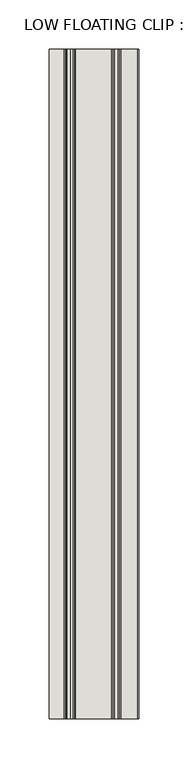
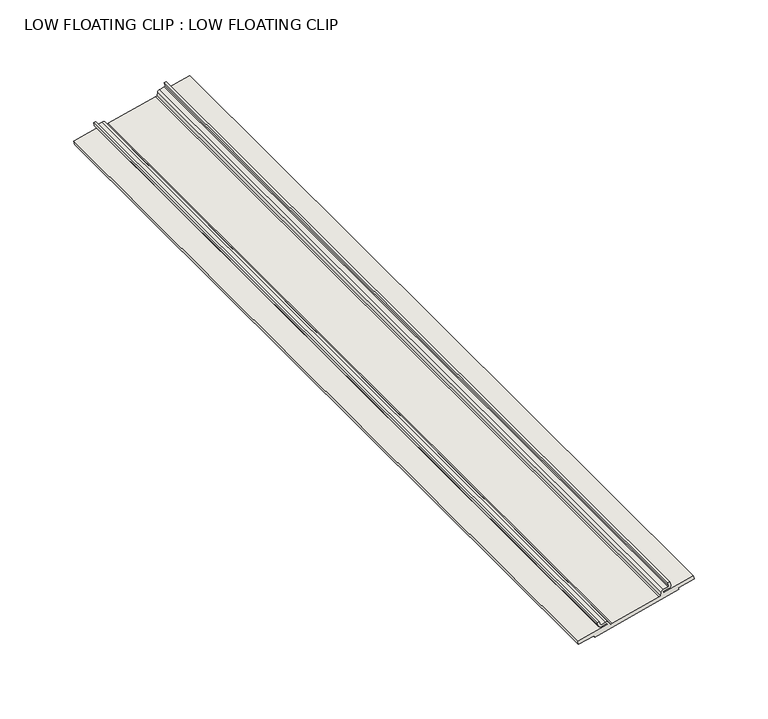
"""IFC4 building model written with IfcOpenShell, lengths in millimetres: wall geometry, LOW FLOATING CLIP : LOW FLOATING CLIP."""

import ifcopenshell
import ifcopenshell.guid

model = None  # the IFC model being written
_history = None  # IfcOwnerHistory: only IFC2X3 demands one
_inside = {}  # id of a spatial element -> (the spatial element, [elements in it])
_under = {}  # id of a project, library or spatial element -> (it, [spatial elements below it])
_declared = {}  # id of a project -> (the project, [libraries it declares])
_typed = {}  # id of a type object -> (the type object, [elements of that type])
_made_of = {}  # id of a material, layer set ... -> (it, [elements and type objects made of it])


def new_model(schema):
    """Start an empty IFC model of exactly this schema.

    Asked for "IFC4X3", IfcOpenShell would pick the latest addendum, in which some entities
    have other attributes; the version numbers below select the first issue.
    IFC2X3 requires an IfcOwnerHistory on every rooted entity: one is made here for all.
    """
    global model, _history
    if schema == "IFC4X3":
        model = ifcopenshell.file(schema_version=(4, 3, 0, 0))
    else:
        model = ifcopenshell.file(schema=schema)
    _inside.clear()
    _under.clear()
    _declared.clear()
    _typed.clear()
    _made_of.clear()
    _history = None
    if model.schema == "IFC2X3":
        org = make("IfcOrganization", Name="unknown")
        user = make(
            "IfcPersonAndOrganization",
            ThePerson=make("IfcPerson", FamilyName="unknown"),
            TheOrganization=org,
        )
        app = make(
            "IfcApplication",
            ApplicationDeveloper=org,
            Version="unknown",
            ApplicationFullName="unknown",
            ApplicationIdentifier="unknown",
        )
        _history = make(
            "IfcOwnerHistory",
            OwningUser=user,
            OwningApplication=app,
            ChangeAction="ADDED",
            CreationDate=0,
        )
    return model


def make(cls, **values):
    """One entity of the class cls with the attributes given. An attribute that is None is left unset."""
    return model.create_entity(
        cls, **{name: value for name, value in values.items() if value is not None}
    )


def rooted(cls, **values):
    """An entity with a GlobalId (a new one), such as an element, a storey or a relation."""
    return make(cls, GlobalId=ifcopenshell.guid.new(), OwnerHistory=_history, **values)


def si_unit(unit_type, name, prefix=None):
    """IfcSIUnit, for example si_unit("LENGTHUNIT", "METRE", prefix="MILLI")."""
    return make("IfcSIUnit", UnitType=unit_type, Prefix=prefix, Name=name)


def assignment(units):
    """IfcUnitAssignment: the units of a project."""
    return None if units is None else make("IfcUnitAssignment", Units=units)


def point(xyz):
    """IfcCartesianPoint."""
    return None if xyz is None else make("IfcCartesianPoint", Coordinates=xyz)


def direction(xyz):
    """IfcDirection."""
    return None if xyz is None else make("IfcDirection", DirectionRatios=xyz)


def frame(location, z_axis=None, x_axis=None):
    """IfcAxis2Placement3D, a coordinate frame: its origin and axes. An axis left out is left unset."""
    return make(
        "IfcAxis2Placement3D",
        Location=point(location),
        Axis=direction(z_axis),
        RefDirection=direction(x_axis),
    )


def origin():
    """The frame at (0, 0, 0) with its axes left unset."""
    return frame((0.0, 0.0, 0.0))


def place(relative_to, where):
    """IfcLocalPlacement: puts the frame where relative to a parent placement (None: the world)."""
    return make(
        "IfcLocalPlacement", PlacementRelTo=relative_to, RelativePlacement=where
    )


def context(
    kind, dimensions, precision=None, world=None, true_north=None, identifier=None
):
    """IfcGeometricRepresentationContext, for example the 3D "Model" context."""
    return make(
        "IfcGeometricRepresentationContext",
        ContextIdentifier=identifier,
        ContextType=kind,
        CoordinateSpaceDimension=dimensions,
        Precision=precision,
        WorldCoordinateSystem=world,
        TrueNorth=true_north,
    )


def project(units=None, contexts=None):
    """IfcProject with its units and contexts."""
    return rooted(
        "IfcProject",
        Name="project",
        RepresentationContexts=contexts,
        UnitsInContext=assignment(units),
    )


def spatial(cls, under=None, at=None, **own):
    """A site, building, storey or space (cls), placed at a placement, below another one or the project."""
    s = rooted(cls, ObjectPlacement=at, **own)
    if under is not None:
        _under.setdefault(under.id(), (under, []))[1].append(s)
    return s


def polyline(points):
    """IfcPolyline through the points."""
    return make("IfcPolyline", Points=[point(p) for p in points])


def circle_curve(where, radius):
    """IfcCircle in the frame where."""
    return make("IfcCircle", Position=where, Radius=radius)


def shape(context_of_items, identifier, shape_type, items):
    """IfcShapeRepresentation: the items that make up one representation, for example the "Body"."""
    return make(
        "IfcShapeRepresentation",
        ContextOfItems=context_of_items,
        RepresentationIdentifier=identifier,
        RepresentationType=shape_type,
        Items=items,
    )


def source(mapping_origin, context_of_items, identifier, shape_type, items):
    """IfcRepresentationMap: a shape defined once, which mapped items show again and again."""
    return make(
        "IfcRepresentationMap",
        MappingOrigin=mapping_origin,
        MappedRepresentation=shape(context_of_items, identifier, shape_type, items),
    )


def transform(
    local_origin,
    x_axis=None,
    y_axis=None,
    z_axis=None,
    scale=None,
    scale2=None,
    scale3=None,
    uniform=True,
):
    """IfcCartesianTransformationOperator3D, or its non-uniform kind. x_axis, y_axis, z_axis: its Axis1, 2, 3."""
    if uniform:
        return make(
            "IfcCartesianTransformationOperator3D",
            Axis1=direction(x_axis),
            Axis2=direction(y_axis),
            LocalOrigin=point(local_origin),
            Scale=scale,
            Axis3=direction(z_axis),
        )
    return make(
        "IfcCartesianTransformationOperator3DnonUniform",
        Axis1=direction(x_axis),
        Axis2=direction(y_axis),
        LocalOrigin=point(local_origin),
        Scale=scale,
        Axis3=direction(z_axis),
        Scale2=scale2,
        Scale3=scale3,
    )


def mapped(mapping_source, mapping_target):
    """IfcMappedItem: shows the shape of a source again, moved by a transform."""
    return make(
        "IfcMappedItem", MappingSource=mapping_source, MappingTarget=mapping_target
    )


def made_of(thing, what):
    """Note that an element or type object is made of a material, layer set ...; save() writes the relation."""
    if what is not None:
        _made_of.setdefault(what.id(), (what, []))[1].append(thing)
    return thing


def element(
    cls,
    number,
    at=None,
    inside=None,
    cuts=None,
    type_object=None,
    material=None,
    context=None,
    identifier="Body",
    shape_type=None,
    held_by="IfcProductDefinitionShape",
    body=None,
    shapes=None,
    **own,
):
    """One element of the class cls, such as IfcWall. Its Tag is "e" and its number.

    at: its placement. inside: the storey or other place that contains it. cuts: it is an
    opening in that element (IfcRelVoidsElement). A single representation is given by context,
    identifier, shape_type and body (its items); several are given by shapes. held_by: the class
    of the entity that holds the representations. save() writes the other relations.
    """
    e = rooted(cls, Tag="e%d" % number, ObjectPlacement=at, **own)
    if body is not None:
        shapes = [shape(context, identifier, shape_type, body)]
    if shapes is not None:
        e.Representation = make(held_by, Representations=shapes)
    if inside is not None:
        _inside.setdefault(inside.id(), (inside, []))[1].append(e)
    if cuts is not None:
        rooted(
            "IfcRelVoidsElement", RelatingBuildingElement=cuts, RelatedOpeningElement=e
        )
    if type_object is not None:
        _typed.setdefault(type_object.id(), (type_object, []))[1].append(e)
    return made_of(e, material)


def aggregate(whole, parts):
    """IfcRelAggregates: a whole, such as a stair, and the parts it consists of."""
    return rooted("IfcRelAggregates", RelatingObject=whole, RelatedObjects=parts)


def save(model, path):
    """Write the relations noted so far, then the file.

    IfcRelAggregates (storeys below a building ...), IfcRelContainedInSpatialStructure (elements
    in a storey), IfcRelDefinesByType, IfcRelAssociatesMaterial and IfcRelDeclares: one each for
    every whole, place, type object, material and project.
    """
    for whole, parts in _under.values():
        aggregate(whole, parts)
    for where, things in _inside.values():
        rooted(
            "IfcRelContainedInSpatialStructure",
            RelatedElements=things,
            RelatingStructure=where,
        )
    for kind, things in _typed.values():
        rooted("IfcRelDefinesByType", RelatedObjects=things, RelatingType=kind)
    for what, things in _made_of.values():
        rooted("IfcRelAssociatesMaterial", RelatedObjects=things, RelatingMaterial=what)
    for by, libraries in _declared.values():
        rooted("IfcRelDeclares", RelatingContext=by, RelatedDefinitions=libraries)
    model.write(path)


def plane_surface(at):
    """IfcPlane: the flat surface through the origin of the frame at, square to its z axis."""
    return make("IfcPlane", Position=at)


def cylinder_surface(at, radius):
    """IfcCylindricalSurface: all points at the distance radius from the z axis of the frame at."""
    return make("IfcCylindricalSurface", Position=at, Radius=radius)


def revolved_surface(curve, axis_point, axis_direction):
    """IfcSurfaceOfRevolution: the curve turned about the line through axis_point along axis_direction."""
    return make(
        "IfcSurfaceOfRevolution",
        SweptCurve=make("IfcArbitraryOpenProfileDef", ProfileType="CURVE", Curve=curve),
        AxisPosition=make("IfcAxis1Placement", Location=point(axis_point), Axis=direction(axis_direction)),
    )


def advanced_brep(points, edges, surfaces, faces):
    """IfcAdvancedBrep: a solid bounded by faces that lie on surfaces and meet in shared edges.

    An edge is (start, end): straight between two places in points (the first is 0);
    or (start, end, curve); or (start, end, curve, False) where it runs against its curve.
    A face is (place in surfaces, loops), or (place, loops, False) where it looks against
    its surface's normal. A loop lists edges by number (the first is 1), with a minus sign
    where the edge is run from its end to its start. The first loop is the outer one.
    """
    corners = [point(p) for p in points]
    vertices = [make("IfcVertexPoint", VertexGeometry=c) for c in corners]
    made = []
    for start, end, *more in edges:
        made.append(
            make(
                "IfcEdgeCurve",
                EdgeStart=vertices[start],
                EdgeEnd=vertices[end],
                EdgeGeometry=more[0] if more else make("IfcPolyline", Points=[corners[start], corners[end]]),
                SameSense=more[1] if len(more) > 1 else True,
            )
        )
    hull = []
    for where, loops, *sense in faces:
        bounds = []
        for j, loop in enumerate(loops):
            ring = [make("IfcOrientedEdge", EdgeElement=made[abs(k) - 1], Orientation=k > 0) for k in loop]
            bounds.append(
                make(
                    "IfcFaceOuterBound" if j == 0 else "IfcFaceBound",
                    Bound=make("IfcEdgeLoop", EdgeList=ring),
                    Orientation=True,
                )
            )
        hull.append(make("IfcAdvancedFace", Bounds=bounds, FaceSurface=surfaces[where], SameSense=sense[0] if sense else True))
    return make("IfcAdvancedBrep", Outer=make("IfcClosedShell", CfsFaces=hull))


def low_floating_clip_low_floating_clip_32a7baed(model_context):
    return source(origin(), model_context, "Body", "AdvancedBrep", [
        advanced_brep(
        [(19368.2427373, -2319.6634634, 2904.7050146), (19368.8587777, -2319.6634634, 2902.2408526), (19371.5072306, -2319.6634634, 2900.6517809), (19375.638583, -2319.6634634, 2901.684619), (19376.3038341, -2319.6634634, 2900.7867945), (19352.6994735, -2319.6634634, 2894.8857043), (19353.3982612, -2319.6634634, 2892.0905533), (19365.7199396, -2319.6634634, 2895.1709729), (19366.0898062, -2319.6634634, 2893.6915066), (19432.0053108, -2319.6634634, 2910.1703828), (19431.6354443, -2319.6634634, 2911.649849), (19443.9571227, -2319.6634634, 2914.7302686), (19443.2583349, -2319.6634634, 2917.5254197), (19419.6539743, -2319.6634634, 2911.6243295), (19419.8184549, -2319.6634634, 2912.729587), (19423.9498072, -2319.6634634, 2913.7624251), (19425.538879, -2319.6634634, 2916.410878), (19424.9228385, -2319.6634634, 2918.8750399), (19423.4448933, -2319.6634634, 2918.5055536), (19424.0609338, -2319.6634634, 2916.0413916), (19423.5794679, -2319.6634634, 2915.2397405), (19419.876029, -2319.6634634, 2914.3138808), (19418.244381, -2319.6634634, 2912.5153002), (19417.8358285, -2319.6634634, 2909.7698187), (19416.7891108, -2319.6634634, 2909.5081393), (19379.827509, -2319.6634634, 2900.2677388), (19378.7807913, -2319.6634634, 2900.0060594), (19377.1283125, -2319.6634634, 2902.236283), (19374.8422323, -2319.6634634, 2903.0554316), (19371.1387933, -2319.6634634, 2902.1295719), (19370.3372749, -2319.6634634, 2902.6104769), (19369.7206825, -2319.6634634, 2905.0745009), (19368.2427373, -1637.0384634, 2904.7050146), (19369.7206825, -1637.0384634, 2905.0745009), (19370.336723, -1637.0384634, 2902.610339), (19371.1387933, -1637.0384634, 2902.1295719), (19374.8422323, -1637.0384634, 2903.0554316), (19377.1283125, -1637.0384634, 2902.236283), (19378.7807913, -1637.0384634, 2900.0060594), (19379.827509, -1637.0384634, 2900.2677388), (19416.7891108, -1637.0384634, 2909.5081393), (19417.8358285, -1637.0384634, 2909.7698187), (19418.244381, -1637.0384634, 2912.5153002), (19419.876029, -1637.0384634, 2914.3138808), (19423.5794679, -1637.0384634, 2915.2397405), (19424.0603818, -1637.0384634, 2916.0412537), (19423.4448933, -1637.0384634, 2918.5055536), (19424.9228385, -1637.0384634, 2918.8750399), (19425.538879, -1637.0384634, 2916.410878), (19423.9498072, -1637.0384634, 2913.7624251), (19419.8184549, -1637.0384634, 2912.729587), (19419.6539743, -1637.0384634, 2911.6243295), (19443.2583349, -1637.0384634, 2917.5254197), (19443.9571227, -1637.0384634, 2914.7302686), (19431.6354443, -1637.0384634, 2911.649849), (19432.0053108, -1637.0384634, 2910.1703828), (19366.0898062, -1637.0384634, 2893.6915066), (19365.7199396, -1637.0384634, 2895.1709729), (19353.3982612, -1637.0384634, 2892.0905533), (19352.6994735, -1637.0384634, 2894.8857043), (19376.3038341, -1637.0384634, 2900.7867945), (19375.638583, -1637.0384634, 2901.684619), (19371.5072306, -1637.0384634, 2900.6517809), (19368.8587777, -1637.0384634, 2902.2408526)],
        [
            (0, 1),
            (1, 2, circle_curve(frame((19370.9775401, -2319.6634634, 2902.7705432), z_axis=(0.0, -1.0, 0.0), x_axis=(-0.9701425001453214, 0.0, -0.24253562503637516)), 2.1839702)),
            (2, 3),
            (3, 4),
            (4, 5),
            (5, 6),
            (6, 7),
            (7, 8),
            (8, 9),
            (9, 10),
            (10, 11),
            (11, 12),
            (12, 13),
            (13, 14),
            (14, 15),
            (15, 16, circle_curve(frame((19423.4201167, -2319.6634634, 2915.8811874), z_axis=(0.0, -1.0, 0.0), x_axis=(0.9701425001453399, 0.0, 0.2425356250363014)), 2.1839702)),
            (16, 17),
            (17, 18),
            (18, 19),
            (19, 20, circle_curve(frame((19423.4191639, -2319.6634634, 2915.8809567), z_axis=(0.0, 1.0, 0.0), x_axis=(0.2425356250361952, 0.0, -0.9701425001453665)), 0.6609505)),
            (20, 21),
            (21, 22, circle_curve(frame((19420.4060948, -2319.6634634, 2912.1936176), z_axis=(0.0, -1.0, 0.0), x_axis=(-0.9891084891577027, 0.0, 0.147188303462493)), 2.1855173)),
            (22, 23),
            (23, 24),
            (24, 25),
            (25, 26),
            (26, 27),
            (27, 28, circle_curve(frame((19375.3722981, -2319.6634634, 2900.9351684), z_axis=(0.0, -1.0, 0.0), x_axis=(0.8034777005685577, 0.0, 0.5953348508940689)), 2.1855173)),
            (28, 29),
            (29, 30, circle_curve(frame((19370.9784893, -2319.6634634, 2902.770788), z_axis=(0.0, 1.0, 0.0), x_axis=(0.2425356250364814, 0.0, -0.9701425001452949)), 0.6609505)),
            (30, 31),
            (31, 0),
            (32, 33),
            (33, 34),
            (34, 35, circle_curve(frame((19370.9784893, -1637.0384634, 2902.770788), z_axis=(0.0, -1.0, 0.0), x_axis=(0.2425356250364814, 0.0, -0.9701425001452949)), 0.6609505)),
            (35, 36),
            (36, 37, circle_curve(frame((19375.3722981, -1637.0384634, 2900.9351684), z_axis=(0.0, 1.0, 0.0), x_axis=(0.8034777005685577, 0.0, 0.5953348508940689)), 2.1855173)),
            (37, 38),
            (38, 39),
            (39, 40),
            (40, 41),
            (41, 42),
            (42, 43, circle_curve(frame((19420.4060948, -1637.0384634, 2912.1936176), z_axis=(0.0, 1.0, 0.0), x_axis=(-0.9891084891577027, 0.0, 0.147188303462493)), 2.1855173)),
            (43, 44),
            (44, 45, circle_curve(frame((19423.4191639, -1637.0384634, 2915.8809567), z_axis=(0.0, -1.0, 0.0), x_axis=(0.2425356250361952, 0.0, -0.9701425001453665)), 0.6609505)),
            (45, 46),
            (46, 47),
            (47, 48),
            (48, 49, circle_curve(frame((19423.4201167, -1637.0384634, 2915.8811874), z_axis=(0.0, 1.0, 0.0), x_axis=(0.9701425001453399, 0.0, 0.2425356250363014)), 2.1839702)),
            (49, 50),
            (50, 51),
            (51, 52),
            (52, 53),
            (53, 54),
            (54, 55),
            (55, 56),
            (56, 57),
            (57, 58),
            (58, 59),
            (59, 60),
            (60, 61),
            (61, 62),
            (62, 63, circle_curve(frame((19370.9775401, -1637.0384634, 2902.7705432), z_axis=(0.0, 1.0, 0.0), x_axis=(-0.9701425001453214, 0.0, -0.24253562503637516)), 2.1839702)),
            (63, 32),
            (0, 32),
            (63, 1),
            (62, 2),
            (61, 3),
            (60, 4),
            (59, 5),
            (58, 6),
            (57, 7),
            (56, 8),
            (55, 9),
            (54, 10),
            (53, 11),
            (52, 12),
            (51, 13),
            (50, 14),
            (49, 15),
            (48, 16),
            (47, 17),
            (46, 18),
            (45, 19),
            (44, 20),
            (43, 21),
            (42, 22),
            (41, 23),
            (40, 24),
            (39, 25),
            (38, 26),
            (37, 27),
            (36, 28),
            (35, 29),
            (34, 30),
            (33, 31),
        ],
        [
            plane_surface(frame((19368.2427373, -2319.6634634, 2904.7050146), z_axis=(0.0, -1.0, 0.0), x_axis=(0.24253562503683454, 0.0, -0.9701425001452065))),
            plane_surface(frame((19368.2427373, -1637.0384634, 2904.7050146), z_axis=(0.0, 1.0, 0.0), x_axis=(-0.24253562503683454, 0.0, 0.9701425001452065))),
            plane_surface(frame((19368.2427373, -2319.6634634, 2904.7050146), z_axis=(-0.9701425001452065, 0.0, -0.24253562503683454), x_axis=(0.0, 1.0, 0.0))),
            cylinder_surface(frame((19370.9775401, -1637.0384634, 2902.7705432), z_axis=(0.0, -1.0000000000000002, 0.0), x_axis=(-0.9701425001453214, 0.0, -0.24253562503637516)), 2.1839702),
            plane_surface(frame((19371.5072306, -2319.6634634, 2900.6517809), z_axis=(0.24253562520086946, 0.0, -0.9701425001041978), x_axis=(0.0, 1.0, 0.0))),
            plane_surface(frame((19375.638583, -2319.6634634, 2901.684619), z_axis=(-0.8034733269729771, 0.0, -0.5953407535546138), x_axis=(0.0, 1.0, 0.0))),
            plane_surface(frame((19376.3038341, -2319.6634634, 2900.7867945), z_axis=(-0.24253562503641676, 0.0, 0.970142500145311), x_axis=(0.0, 1.0, 0.0))),
            plane_surface(frame((19352.6994735, -2319.6634634, 2894.8857043), z_axis=(-0.9701425001452767, 0.0, -0.24253562503655407), x_axis=(0.0, 1.0, 0.0))),
            plane_surface(frame((19353.3982612, -2319.6634634, 2892.0905533), z_axis=(0.24253562503641324, 0.0, -0.9701425001453119), x_axis=(0.0, 1.0, 0.0))),
            plane_surface(frame((19365.7199396, -2319.6634634, 2895.1709729), z_axis=(-0.9701425001450604, 0.0, -0.242535625037419), x_axis=(0.0, 1.0, 0.0))),
            plane_surface(frame((19366.0898062, -2319.6634634, 2893.6915066), z_axis=(0.24253562503641551, 0.0, -0.9701425001453113), x_axis=(0.0, 1.0, 0.0))),
            plane_surface(frame((19432.0053108, -2319.6634634, 2910.1703828), z_axis=(0.9701425001452693, 0.0, 0.2425356250365836), x_axis=(0.0, 1.0, 0.0))),
            plane_surface(frame((19431.6354443, -2319.6634634, 2911.649849), z_axis=(0.24253562503625273, 0.0, -0.970142500145352), x_axis=(0.0, 1.0, 0.0))),
            plane_surface(frame((19443.9571227, -2319.6634634, 2914.7302686), z_axis=(0.9701425001452103, 0.0, 0.24253562503681939), x_axis=(0.0, 1.0, 0.0))),
            plane_surface(frame((19443.2583349, -2319.6634634, 2917.5254197), z_axis=(-0.24253562503627013, 0.0, 0.9701425001453476), x_axis=(0.0, 1.0, 0.0))),
            plane_surface(frame((19419.6539743, -2319.6634634, 2911.6243295), z_axis=(0.9891074078253219, 0.0, -0.14719556985545568), x_axis=(0.0, 1.0, 0.0))),
            plane_surface(frame((19419.8184549, -2319.6634634, 2912.729587), z_axis=(0.24253562503621331, 0.0, -0.9701425001453619), x_axis=(0.0, 1.0, 0.0))),
            cylinder_surface(frame((19423.4201167, -1637.0384634, 2915.8811874), z_axis=(0.0, -1.0000000000000002, 0.0), x_axis=(0.9701425001453399, 0.0, 0.2425356250363014)), 2.1839702),
            plane_surface(frame((19425.538879, -2319.6634634, 2916.410878), z_axis=(0.97014250014631, 0.0, 0.24253562503242082), x_axis=(0.0, 1.0, 0.0))),
            plane_surface(frame((19424.9228385, -2319.6634634, 2918.8750399), z_axis=(-0.24253562503633297, 0.0, 0.9701425001453319), x_axis=(0.0, 1.0, 0.0))),
            plane_surface(frame((19423.4448933, -2319.6634634, 2918.5055536), z_axis=(-0.9701425001454071, 0.0, -0.24253562503603204), x_axis=(0.0, 1.0, 0.0))),
            revolved_surface(polyline([(19423.579467942633, -1637.0384634, 2915.2397405294573), (19423.579467942633, -2319.6634634, 2915.2397405294573)]), (19423.4191639, -1637.0384634, 2915.8809567), (0.0, 1.0000000000000002, 0.0)),
            plane_surface(frame((19423.5794679, -2319.6634634, 2915.2397405), z_axis=(-0.242535625035799, 0.0, 0.9701425001454654), x_axis=(0.0, 1.0, 0.0))),
            cylinder_surface(frame((19420.4060948, -1637.0384634, 2912.1936176), z_axis=(0.0, -1.0, 0.0), x_axis=(-0.9891084891577027, 0.0, 0.147188303462493)), 2.1855173),
            plane_surface(frame((19418.244381, -2319.6634634, 2912.5153002), z_axis=(-0.9891084891587392, 0.0, 0.1471883034555279), x_axis=(0.0, 1.0, 0.0))),
            plane_surface(frame((19417.8358285, -2319.6634634, 2909.7698187), z_axis=(-0.24253562503586068, 0.0, 0.97014250014545), x_axis=(0.0, 1.0, 0.0))),
            plane_surface(frame((19416.7891108, -2319.6634634, 2909.5081393), z_axis=(-0.24253562503634635, 0.0, 0.9701425001453285), x_axis=(0.0, 1.0, 0.0))),
            plane_surface(frame((19379.827509, -2319.6634634, 2900.2677388), z_axis=(-0.24253562503633297, 0.0, 0.9701425001453319), x_axis=(0.0, 1.0, 0.0))),
            plane_surface(frame((19378.7807913, -2319.6634634, 2900.0060594), z_axis=(0.8034777005687778, 0.0, 0.5953348508937718), x_axis=(0.0, 1.0, 0.0))),
            cylinder_surface(frame((19375.3722981, -1637.0384634, 2900.9351684), z_axis=(0.0, -1.0000000000000002, 0.0), x_axis=(0.8034777005685577, 0.0, 0.5953348508940689)), 2.1855173),
            plane_surface(frame((19374.8422323, -2319.6634634, 2903.0554316), z_axis=(-0.24253562742045254, 0.0, 0.9701424995493021), x_axis=(0.0, 1.0, 0.0))),
            revolved_surface(polyline([(19371.138793342634, -1637.0384634, 2902.1295718294577), (19371.138793342634, -2319.6634634, 2902.1295718294577)]), (19370.9784893, -1637.0384634, 2902.770788), (0.0, 1.0000000000000002, 0.0)),
            plane_surface(frame((19370.336723, -2319.6634634, 2902.610339), z_axis=(0.9701425001453114, 0.0, 0.2425356250364152), x_axis=(0.0, 1.0, 0.0))),
            plane_surface(frame((19369.7206825, -2319.6634634, 2905.0745009), z_axis=(-0.24253562503633297, 0.0, 0.9701425001453319), x_axis=(0.0, 1.0, 0.0))),
        ],
        [
            (0, [[1, 2, 3, 4, 5, 6, 7, 8, 9, 10, 11, 12, 13, 14, 15, 16, 17, 18, 19, 20, 21, 22, 23, 24, 25, 26, 27, 28, 29, 30, 31, 32]]),
            (1, [[33, 34, 35, 36, 37, 38, 39, 40, 41, 42, 43, 44, 45, 46, 47, 48, 49, 50, 51, 52, 53, 54, 55, 56, 57, 58, 59, 60, 61, 62, 63, 64]]),
            (2, [[-1, 65, -64, 66]]),
            (3, [[-2, -66, -63, 67]]),
            (4, [[-3, -67, -62, 68]]),
            (5, [[-4, -68, -61, 69]]),
            (6, [[-5, -69, -60, 70]]),
            (7, [[-6, -70, -59, 71]]),
            (8, [[-7, -71, -58, 72]]),
            (9, [[-8, -72, -57, 73]]),
            (10, [[-9, -73, -56, 74]]),
            (11, [[-10, -74, -55, 75]]),
            (12, [[-11, -75, -54, 76]]),
            (13, [[-12, -76, -53, 77]]),
            (14, [[-13, -77, -52, 78]]),
            (15, [[-14, -78, -51, 79]]),
            (16, [[-15, -79, -50, 80]]),
            (17, [[-16, -80, -49, 81]]),
            (18, [[-17, -81, -48, 82]]),
            (19, [[-18, -82, -47, 83]]),
            (20, [[-19, -83, -46, 84]]),
            (21, [[-20, -84, -45, 85]]),
            (22, [[-21, -85, -44, 86]]),
            (23, [[-22, -86, -43, 87]]),
            (24, [[-23, -87, -42, 88]]),
            (25, [[-24, -88, -41, 89]]),
            (26, [[-25, -89, -40, 90]]),
            (27, [[-26, -90, -39, 91]]),
            (28, [[-27, -91, -38, 92]]),
            (29, [[-28, -92, -37, 93]]),
            (30, [[-29, -93, -36, 94]]),
            (31, [[-30, -94, -35, 95]]),
            (32, [[-31, -95, -34, 96]]),
            (33, [[-32, -96, -33, -65]]),
        ],
    ),
    ])


if __name__ == "__main__":
    model = new_model("IFC4")
    model_context = context("Model", 3, world=origin())
    ifc_project = project(units=[si_unit("LENGTHUNIT", "METRE", prefix="MILLI")], contexts=[model_context])
    site = spatial("IfcSite", under=ifc_project)
    building = spatial("IfcBuilding", under=site)
    placement = place(None, origin())
    low_floating_clip_low_floating_clip_shape = low_floating_clip_low_floating_clip_32a7baed(model_context)
    element("IfcWall", 1, ObjectType="LOW FLOATING CLIP : LOW FLOATING CLIP", at=placement, inside=building, context=model_context, shape_type="MappedRepresentation", body=[
        mapped(low_floating_clip_low_floating_clip_shape, transform((0.0, 0.0, 0.0), x_axis=(1.0, 0.0, 0.0), y_axis=(0.0, 1.0, 0.0), z_axis=(0.0, 0.0, 1.0))),
    ])
    save(model, "model.ifc")

# Revit data of these elements
# Element 1 (IfcWall, "LOW FLOATING CLIP : LOW FLOATING CLIP")
#   Materials on its faces: "LOW FLOATING CLIP"
# Materials
#   "LOW FLOATING CLIP": class "Metal", colour RGB 247 247 247, transparency 0, Cost = 0
